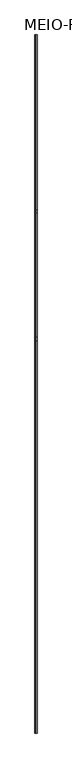
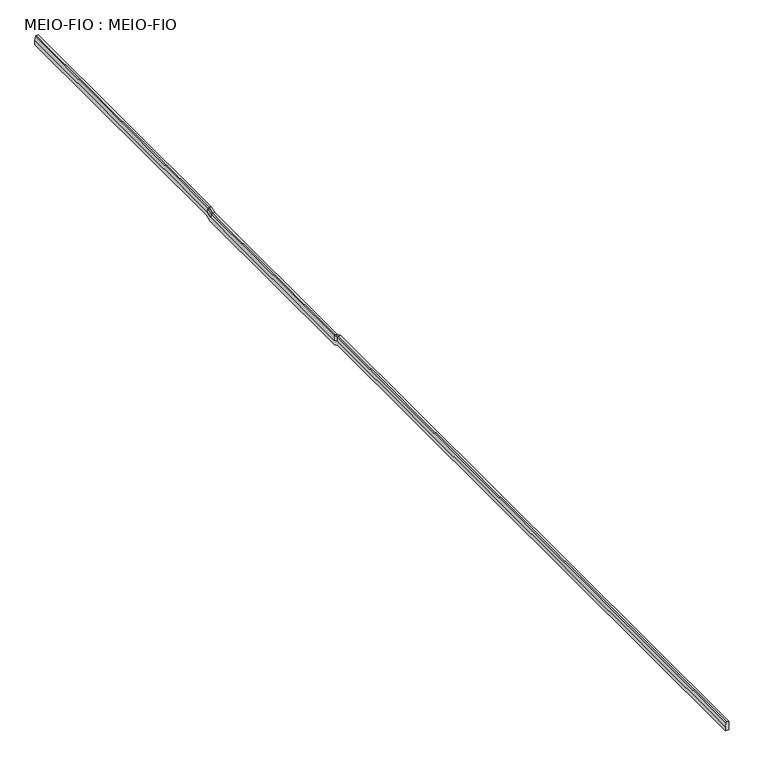
"""IFC4 building model written with IfcOpenShell, lengths in millimetres: proxy geometry, MEIO-FIO : MEIO-FIO."""

import ifcopenshell
import ifcopenshell.guid

model = None  # the IFC model being written
_history = None  # IfcOwnerHistory: only IFC2X3 demands one
_inside = {}  # id of a spatial element -> (the spatial element, [elements in it])
_under = {}  # id of a project, library or spatial element -> (it, [spatial elements below it])
_declared = {}  # id of a project -> (the project, [libraries it declares])
_typed = {}  # id of a type object -> (the type object, [elements of that type])
_made_of = {}  # id of a material, layer set ... -> (it, [elements and type objects made of it])


def new_model(schema):
    """Start an empty IFC model of exactly this schema.

    Asked for "IFC4X3", IfcOpenShell would pick the latest addendum, in which some entities
    have other attributes; the version numbers below select the first issue.
    IFC2X3 requires an IfcOwnerHistory on every rooted entity: one is made here for all.
    """
    global model, _history
    if schema == "IFC4X3":
        model = ifcopenshell.file(schema_version=(4, 3, 0, 0))
    else:
        model = ifcopenshell.file(schema=schema)
    _inside.clear()
    _under.clear()
    _declared.clear()
    _typed.clear()
    _made_of.clear()
    _history = None
    if model.schema == "IFC2X3":
        org = make("IfcOrganization", Name="unknown")
        user = make(
            "IfcPersonAndOrganization",
            ThePerson=make("IfcPerson", FamilyName="unknown"),
            TheOrganization=org,
        )
        app = make(
            "IfcApplication",
            ApplicationDeveloper=org,
            Version="unknown",
            ApplicationFullName="unknown",
            ApplicationIdentifier="unknown",
        )
        _history = make(
            "IfcOwnerHistory",
            OwningUser=user,
            OwningApplication=app,
            ChangeAction="ADDED",
            CreationDate=0,
        )
    return model


def make(cls, **values):
    """One entity of the class cls with the attributes given. An attribute that is None is left unset."""
    return model.create_entity(
        cls, **{name: value for name, value in values.items() if value is not None}
    )


def rooted(cls, **values):
    """An entity with a GlobalId (a new one), such as an element, a storey or a relation."""
    return make(cls, GlobalId=ifcopenshell.guid.new(), OwnerHistory=_history, **values)


def si_unit(unit_type, name, prefix=None):
    """IfcSIUnit, for example si_unit("LENGTHUNIT", "METRE", prefix="MILLI")."""
    return make("IfcSIUnit", UnitType=unit_type, Prefix=prefix, Name=name)


def assignment(units):
    """IfcUnitAssignment: the units of a project."""
    return None if units is None else make("IfcUnitAssignment", Units=units)


def point(xyz):
    """IfcCartesianPoint."""
    return None if xyz is None else make("IfcCartesianPoint", Coordinates=xyz)


def direction(xyz):
    """IfcDirection."""
    return None if xyz is None else make("IfcDirection", DirectionRatios=xyz)


def frame(location, z_axis=None, x_axis=None):
    """IfcAxis2Placement3D, a coordinate frame: its origin and axes. An axis left out is left unset."""
    return make(
        "IfcAxis2Placement3D",
        Location=point(location),
        Axis=direction(z_axis),
        RefDirection=direction(x_axis),
    )


def origin():
    """The frame at (0, 0, 0) with its axes left unset."""
    return frame((0.0, 0.0, 0.0))


def place(relative_to, where):
    """IfcLocalPlacement: puts the frame where relative to a parent placement (None: the world)."""
    return make(
        "IfcLocalPlacement", PlacementRelTo=relative_to, RelativePlacement=where
    )


def context(
    kind, dimensions, precision=None, world=None, true_north=None, identifier=None
):
    """IfcGeometricRepresentationContext, for example the 3D "Model" context."""
    return make(
        "IfcGeometricRepresentationContext",
        ContextIdentifier=identifier,
        ContextType=kind,
        CoordinateSpaceDimension=dimensions,
        Precision=precision,
        WorldCoordinateSystem=world,
        TrueNorth=true_north,
    )


def project(units=None, contexts=None):
    """IfcProject with its units and contexts."""
    return rooted(
        "IfcProject",
        Name="project",
        RepresentationContexts=contexts,
        UnitsInContext=assignment(units),
    )


def spatial(cls, under=None, at=None, **own):
    """A site, building, storey or space (cls), placed at a placement, below another one or the project."""
    s = rooted(cls, ObjectPlacement=at, **own)
    if under is not None:
        _under.setdefault(under.id(), (under, []))[1].append(s)
    return s


def circle_curve(where, radius):
    """IfcCircle in the frame where."""
    return make("IfcCircle", Position=where, Radius=radius)


def ellipse_curve(where, semi_axis1, semi_axis2):
    """IfcEllipse in the frame where."""
    return make(
        "IfcEllipse", Position=where, SemiAxis1=semi_axis1, SemiAxis2=semi_axis2
    )


def shape(context_of_items, identifier, shape_type, items):
    """IfcShapeRepresentation: the items that make up one representation, for example the "Body"."""
    return make(
        "IfcShapeRepresentation",
        ContextOfItems=context_of_items,
        RepresentationIdentifier=identifier,
        RepresentationType=shape_type,
        Items=items,
    )


def source(mapping_origin, context_of_items, identifier, shape_type, items):
    """IfcRepresentationMap: a shape defined once, which mapped items show again and again."""
    return make(
        "IfcRepresentationMap",
        MappingOrigin=mapping_origin,
        MappedRepresentation=shape(context_of_items, identifier, shape_type, items),
    )


def transform(
    local_origin,
    x_axis=None,
    y_axis=None,
    z_axis=None,
    scale=None,
    scale2=None,
    scale3=None,
    uniform=True,
):
    """IfcCartesianTransformationOperator3D, or its non-uniform kind. x_axis, y_axis, z_axis: its Axis1, 2, 3."""
    if uniform:
        return make(
            "IfcCartesianTransformationOperator3D",
            Axis1=direction(x_axis),
            Axis2=direction(y_axis),
            LocalOrigin=point(local_origin),
            Scale=scale,
            Axis3=direction(z_axis),
        )
    return make(
        "IfcCartesianTransformationOperator3DnonUniform",
        Axis1=direction(x_axis),
        Axis2=direction(y_axis),
        LocalOrigin=point(local_origin),
        Scale=scale,
        Axis3=direction(z_axis),
        Scale2=scale2,
        Scale3=scale3,
    )


def mapped(mapping_source, mapping_target):
    """IfcMappedItem: shows the shape of a source again, moved by a transform."""
    return make(
        "IfcMappedItem", MappingSource=mapping_source, MappingTarget=mapping_target
    )


def made_of(thing, what):
    """Note that an element or type object is made of a material, layer set ...; save() writes the relation."""
    if what is not None:
        _made_of.setdefault(what.id(), (what, []))[1].append(thing)
    return thing


def element(
    cls,
    number,
    at=None,
    inside=None,
    cuts=None,
    type_object=None,
    material=None,
    context=None,
    identifier="Body",
    shape_type=None,
    held_by="IfcProductDefinitionShape",
    body=None,
    shapes=None,
    **own,
):
    """One element of the class cls, such as IfcWall. Its Tag is "e" and its number.

    at: its placement. inside: the storey or other place that contains it. cuts: it is an
    opening in that element (IfcRelVoidsElement). A single representation is given by context,
    identifier, shape_type and body (its items); several are given by shapes. held_by: the class
    of the entity that holds the representations. save() writes the other relations.
    """
    e = rooted(cls, Tag="e%d" % number, ObjectPlacement=at, **own)
    if body is not None:
        shapes = [shape(context, identifier, shape_type, body)]
    if shapes is not None:
        e.Representation = make(held_by, Representations=shapes)
    if inside is not None:
        _inside.setdefault(inside.id(), (inside, []))[1].append(e)
    if cuts is not None:
        rooted(
            "IfcRelVoidsElement", RelatingBuildingElement=cuts, RelatedOpeningElement=e
        )
    if type_object is not None:
        _typed.setdefault(type_object.id(), (type_object, []))[1].append(e)
    return made_of(e, material)


def aggregate(whole, parts):
    """IfcRelAggregates: a whole, such as a stair, and the parts it consists of."""
    return rooted("IfcRelAggregates", RelatingObject=whole, RelatedObjects=parts)


def save(model, path):
    """Write the relations noted so far, then the file.

    IfcRelAggregates (storeys below a building ...), IfcRelContainedInSpatialStructure (elements
    in a storey), IfcRelDefinesByType, IfcRelAssociatesMaterial and IfcRelDeclares: one each for
    every whole, place, type object, material and project.
    """
    for whole, parts in _under.values():
        aggregate(whole, parts)
    for where, things in _inside.values():
        rooted(
            "IfcRelContainedInSpatialStructure",
            RelatedElements=things,
            RelatingStructure=where,
        )
    for kind, things in _typed.values():
        rooted("IfcRelDefinesByType", RelatedObjects=things, RelatingType=kind)
    for what, things in _made_of.values():
        rooted("IfcRelAssociatesMaterial", RelatedObjects=things, RelatingMaterial=what)
    for by, libraries in _declared.values():
        rooted("IfcRelDeclares", RelatingContext=by, RelatedDefinitions=libraries)
    model.write(path)


def plane_surface(at):
    """IfcPlane: the flat surface through the origin of the frame at, square to its z axis."""
    return make("IfcPlane", Position=at)


def cylinder_surface(at, radius):
    """IfcCylindricalSurface: all points at the distance radius from the z axis of the frame at."""
    return make("IfcCylindricalSurface", Position=at, Radius=radius)


def advanced_brep(points, edges, surfaces, faces):
    """IfcAdvancedBrep: a solid bounded by faces that lie on surfaces and meet in shared edges.

    An edge is (start, end): straight between two places in points (the first is 0);
    or (start, end, curve); or (start, end, curve, False) where it runs against its curve.
    A face is (place in surfaces, loops), or (place, loops, False) where it looks against
    its surface's normal. A loop lists edges by number (the first is 1), with a minus sign
    where the edge is run from its end to its start. The first loop is the outer one.
    """
    corners = [point(p) for p in points]
    vertices = [make("IfcVertexPoint", VertexGeometry=c) for c in corners]
    made = []
    for start, end, *more in edges:
        made.append(
            make(
                "IfcEdgeCurve",
                EdgeStart=vertices[start],
                EdgeEnd=vertices[end],
                EdgeGeometry=more[0] if more else make("IfcPolyline", Points=[corners[start], corners[end]]),
                SameSense=more[1] if len(more) > 1 else True,
            )
        )
    hull = []
    for where, loops, *sense in faces:
        bounds = []
        for j, loop in enumerate(loops):
            ring = [make("IfcOrientedEdge", EdgeElement=made[abs(k) - 1], Orientation=k > 0) for k in loop]
            bounds.append(
                make(
                    "IfcFaceOuterBound" if j == 0 else "IfcFaceBound",
                    Bound=make("IfcEdgeLoop", EdgeList=ring),
                    Orientation=True,
                )
            )
        hull.append(make("IfcAdvancedFace", Bounds=bounds, FaceSurface=surfaces[where], SameSense=sense[0] if sense else True))
    return make("IfcAdvancedBrep", Outer=make("IfcClosedShell", CfsFaces=hull))


def meio_fio_meio_fio_c5939b1e(model_context):
    return source(origin(), model_context, "Body", "AdvancedBrep", [
        advanced_brep(
        [(-19460.281307, 17327.5225294, 100.0), (-19460.281307, 17327.5225294, -200.0), (-19580.281307, 17327.5225294, -200.0), (-19580.281307, 17327.5225294, -50.0), (-19560.334366, 17327.5225294, 74.7371665), (-19530.7107394, 17327.5225294, 100.0), (-19460.281307, 7304.4300153, 100.0), (-19460.281307, 7104.4300153, 20.0), (-19460.281307, 4.4300153, 20.0), (-19460.281307, -195.5699847, 100.0), (-19460.281307, -22700.938406, 100.0), (-19460.281307, -22700.938406, -200.0), (-19460.281307, -253.3447058, -200.0), (-19460.281307, -53.3447058, -280.0), (-19460.281307, 7162.2047364, -280.0), (-19460.281307, 7362.2047364, -200.0), (-19580.281307, 7362.2047364, -200.0), (-19580.281307, 7162.2047364, -280.0), (-19580.281307, -53.3447058, -280.0), (-19580.281307, -253.3447058, -200.0), (-19580.281307, -22700.938406, -200.0), (-19580.281307, -22700.938406, -50.0), (-19580.281307, -224.4573452, -50.0), (-19580.281307, -24.4573452, -130.0), (-19580.281307, 7133.3173758, -130.0), (-19580.281307, 7333.3173758, -50.0), (-19560.334366, 7309.2951925, 74.7371665), (-19530.7107394, 7304.4300153, 100.0), (-19560.334366, 7109.2951925, -5.2628335), (-19530.7107394, 7104.4300153, 20.0), (-19560.334366, -0.4351619, -5.2628335), (-19530.7107394, 4.4300153, 20.0), (-19560.334366, -200.4351619, 74.7371665), (-19530.7107394, -195.5699847, 100.0), (-19530.7107394, -22700.938406, 100.0), (-19560.334366, -22700.938406, 74.7371665)],
        [
            (0, 1),
            (1, 2),
            (2, 3),
            (3, 4),
            (4, 5, circle_curve(frame((-19530.7107394, 17327.5225294, 70.0), z_axis=(0.0, 1.0, 0.0), x_axis=(-1.0, 0.0, 0.0)), 30.0)),
            (5, 0),
            (0, 6),
            (6, 7),
            (7, 8),
            (8, 9),
            (9, 10),
            (10, 11),
            (11, 12),
            (12, 13),
            (13, 14),
            (14, 15),
            (15, 1),
            (15, 16),
            (16, 2),
            (16, 17),
            (17, 18),
            (18, 19),
            (19, 20),
            (20, 21),
            (21, 22),
            (22, 23),
            (23, 24),
            (24, 25),
            (25, 3),
            (25, 26),
            (26, 4),
            (26, 27, ellipse_curve(frame((-19530.7107394, 7310.2074874, 70.0), z_axis=(0.0, 0.9819563867314226, 0.18910752115494767), x_axis=(0.0, 0.18910752115494667, -0.9819563867314226)), 30.551255, 30.0)),
            (27, 5),
            (27, 6),
            (14, 17),
            (24, 28),
            (28, 26),
            (28, 29, ellipse_curve(frame((-19530.7107394, 7110.2074874, -10.0), z_axis=(0.0, 0.9819563867314226, 0.18910752115494764), x_axis=(0.0, -0.18910752115494842, 0.9819563867314223)), 30.551255, 30.0)),
            (29, 27),
            (29, 7),
            (13, 18),
            (23, 30),
            (30, 28),
            (30, 31, ellipse_curve(frame((-19530.7107394, -1.3474568, -10.0), z_axis=(0.0, 0.9819563867314217, -0.1891075211549513), x_axis=(0.0, 0.18910752115495252, 0.9819563867314217)), 30.551255, 30.0)),
            (31, 29),
            (31, 8),
            (12, 19),
            (22, 32),
            (32, 30),
            (32, 33, ellipse_curve(frame((-19530.7107394, -201.3474568, 70.0), z_axis=(0.0, 0.9819563867314217, -0.18910752115495139), x_axis=(0.0, -0.18910752115495078, -0.9819563867314218)), 30.551255, 30.0)),
            (33, 31),
            (33, 9),
            (10, 34),
            (34, 35, circle_curve(frame((-19530.7107394, -22700.938406, 70.0), z_axis=(0.0, -1.0, 0.0), x_axis=(-1.0, 0.0, 0.0)), 30.0)),
            (35, 21),
            (20, 11),
            (35, 32),
            (34, 33),
        ],
        [
            plane_surface(frame((-19460.281307, 17327.5225294, 100.0), z_axis=(0.0, 1.0, 0.0), x_axis=(0.0, 0.0, 1.0))),
            plane_surface(frame((-19460.281307, 17327.5225294, 100.0), z_axis=(1.0, 0.0, 0.0), x_axis=(0.0, -1.0, 0.0))),
            plane_surface(frame((-19460.281307, 17327.5225294, -200.0), z_axis=(0.0, 0.0, -1.0), x_axis=(0.0, -1.0, 0.0))),
            plane_surface(frame((-19580.281307, 17327.5225294, -200.0), z_axis=(-1.0, 0.0, 0.0), x_axis=(0.0, -1.0, 0.0))),
            plane_surface(frame((-19580.281307, 17327.5225294, -50.0), z_axis=(-0.9874542202157147, 0.0, 0.15790555081495689), x_axis=(0.0, -1.0, 0.0))),
            cylinder_surface(frame((-19530.7107394, 17327.5225294, 70.0), z_axis=(0.0, 1.0, 0.0), x_axis=(-1.0, 0.0, 0.0)), 30.0),
            plane_surface(frame((-19530.7107394, 17327.5225294, 100.0), z_axis=(0.0, 0.0, 1.0), x_axis=(0.0, -1.0, 0.0))),
            plane_surface(frame((-19460.281307, 7362.2047364, -200.0), z_axis=(0.0, 0.3713906763540969, -0.9284766908852621), x_axis=(0.0, -0.9284766908852621, -0.3713906763540969))),
            plane_surface(frame((-19580.281307, 7333.3173758, -50.0), z_axis=(-0.9874542202157147, -0.05864464931723302, 0.1466116232930858), x_axis=(0.0, -0.9284766908852622, -0.3713906763540966))),
            cylinder_surface(frame((-19530.7107394, 7315.5717356, 72.1456993), z_axis=(0.0, 0.9284766908852621, 0.3713906763540969), x_axis=(-1.0, 0.0, 0.0)), 30.0),
            plane_surface(frame((-19530.7107394, 7304.4300153, 100.0), z_axis=(0.0, -0.37139067635409667, 0.9284766908852622), x_axis=(0.0, -0.9284766908852622, -0.37139067635409667))),
            plane_surface(frame((-19460.281307, 7162.2047364, -280.0), z_axis=(0.0, 0.0, -1.0), x_axis=(0.0, -1.0, 0.0))),
            plane_surface(frame((-19580.281307, 7133.3173758, -130.0), z_axis=(-0.9874542202157146, 0.0, 0.15790555081495686), x_axis=(0.0, -1.0, 0.0))),
            cylinder_surface(frame((-19530.7107394, 7104.4300153, -10.0), z_axis=(0.0, 1.0, 0.0), x_axis=(-1.0, 0.0, 0.0)), 30.0),
            plane_surface(frame((-19530.7107394, 7104.4300153, 20.0), z_axis=(0.0, 0.0, 1.0), x_axis=(0.0, -1.0, 0.0))),
            plane_surface(frame((-19460.281307, -53.3447058, -280.0), z_axis=(0.0, -0.37139067635410367, -0.9284766908852594), x_axis=(0.0, -0.9284766908852594, 0.37139067635410367))),
            plane_surface(frame((-19580.281307, -24.4573452, -130.0), z_axis=(-0.9874542202157147, 0.05864464931723411, 0.14661162329308536), x_axis=(0.0, -0.9284766908852594, 0.37139067635410355))),
            cylinder_surface(frame((-19530.7107394, -6.711705, -7.8543007), z_axis=(0.0, 0.9284766908852593, -0.3713906763541038), x_axis=(-1.0, 0.0, 0.0)), 30.0),
            plane_surface(frame((-19530.7107394, 4.4300153, 20.0), z_axis=(0.0, 0.3713906763541038, 0.9284766908852593), x_axis=(0.0, -0.9284766908852593, 0.3713906763541038))),
            plane_surface(frame((-19460.281307, -22700.938406, 100.0), z_axis=(0.0, -1.0, 0.0), x_axis=(0.0, 0.0, 1.0))),
            plane_surface(frame((-19460.281307, -253.3447058, -200.0), z_axis=(0.0, 0.0, -1.0), x_axis=(0.0, -1.0, 0.0))),
            plane_surface(frame((-19580.281307, -224.4573452, -50.0), z_axis=(-0.9874542202157146, 0.0, 0.15790555081495683), x_axis=(0.0, -1.0, 0.0))),
            cylinder_surface(frame((-19530.7107394, -195.5699847, 70.0), z_axis=(0.0, 1.0, 0.0), x_axis=(-1.0, 0.0, 0.0)), 30.0),
            plane_surface(frame((-19530.7107394, -195.5699847, 100.0), z_axis=(0.0, 0.0, 1.0), x_axis=(0.0, -1.0, 0.0))),
        ],
        [
            (0, [[1, 2, 3, 4, 5, 6]]),
            (1, [[-1, 7, 8, 9, 10, 11, 12, 13, 14, 15, 16, 17]]),
            (2, [[-2, -17, 18, 19]]),
            (3, [[-3, -19, 20, 21, 22, 23, 24, 25, 26, 27, 28, 29]]),
            (4, [[-4, -29, 30, 31]]),
            (5, [[-5, -31, 32, 33]]),
            (6, [[-6, -33, 34, -7]]),
            (7, [[-18, -16, 35, -20]]),
            (8, [[-30, -28, 36, 37]]),
            (9, [[-32, -37, 38, 39]]),
            (10, [[-34, -39, 40, -8]]),
            (11, [[-35, -15, 41, -21]]),
            (12, [[-36, -27, 42, 43]]),
            (13, [[-38, -43, 44, 45]]),
            (14, [[-40, -45, 46, -9]]),
            (15, [[-41, -14, 47, -22]]),
            (16, [[-42, -26, 48, 49]]),
            (17, [[-44, -49, 50, 51]]),
            (18, [[-46, -51, 52, -10]]),
            (19, [[53, 54, 55, -24, 56, -12]]),
            (20, [[-47, -13, -56, -23]]),
            (21, [[-48, -25, -55, 57]]),
            (22, [[-50, -57, -54, 58]]),
            (23, [[-52, -58, -53, -11]]),
        ],
    ),
    ])


if __name__ == "__main__":
    model = new_model("IFC4")
    model_context = context("Model", 3, world=origin())
    ifc_project = project(units=[si_unit("LENGTHUNIT", "METRE", prefix="MILLI")], contexts=[model_context])
    site = spatial("IfcSite", under=ifc_project)
    building = spatial("IfcBuilding", under=site)
    placement = place(None, origin())
    meio_fio_meio_fio_shape = meio_fio_meio_fio_c5939b1e(model_context)
    element("IfcBuildingElementProxy", 1, Name="MEIO-FIO : MEIO-FIO", ObjectType="MEIO-FIO : MEIO-FIO", at=placement, inside=building, context=model_context, shape_type="MappedRepresentation", body=[
        mapped(meio_fio_meio_fio_shape, transform((0.0, 0.0, 0.0), x_axis=(1.0, 0.0, 0.0), y_axis=(0.0, 1.0, 0.0), z_axis=(0.0, 0.0, 1.0))),
    ])
    save(model, "model.ifc")

# Revit data of these elements
# Element 1 (IfcBuildingElementProxy, "MEIO-FIO : MEIO-FIO")
#   Materials on its faces: ".PAVIMENTAÇÃO CALÇADA"
# Materials
#   ".PAVIMENTAÇÃO CALÇADA": class ".CC_PAVIMENTAÇÃO", colour RGB 176 176 176, transparency 0, Description = "Pavimentação calçada cinza claro", Cost = 0
